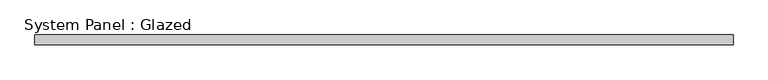
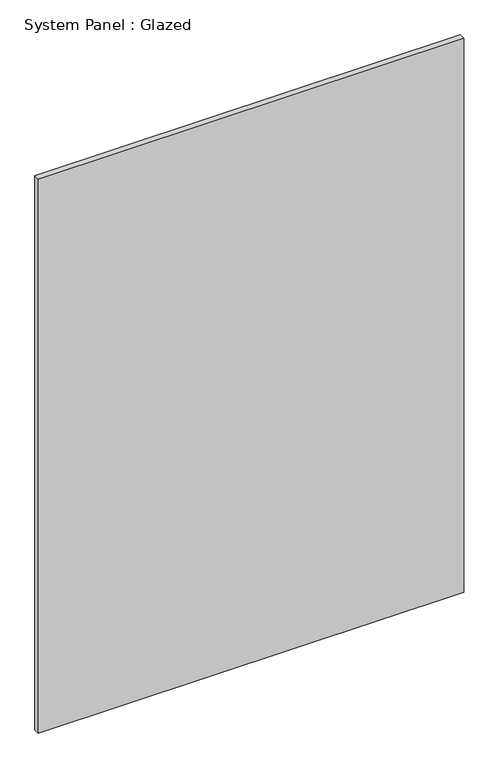
"""IFC4 building model written with IfcOpenShell, lengths in millimetres: plate geometry, System Panel : Glazed."""

import ifcopenshell
import ifcopenshell.guid

model = None  # the IFC model being written
_history = None  # IfcOwnerHistory: only IFC2X3 demands one
_inside = {}  # id of a spatial element -> (the spatial element, [elements in it])
_under = {}  # id of a project, library or spatial element -> (it, [spatial elements below it])
_declared = {}  # id of a project -> (the project, [libraries it declares])
_typed = {}  # id of a type object -> (the type object, [elements of that type])
_made_of = {}  # id of a material, layer set ... -> (it, [elements and type objects made of it])


def new_model(schema):
    """Start an empty IFC model of exactly this schema.

    Asked for "IFC4X3", IfcOpenShell would pick the latest addendum, in which some entities
    have other attributes; the version numbers below select the first issue.
    IFC2X3 requires an IfcOwnerHistory on every rooted entity: one is made here for all.
    """
    global model, _history
    if schema == "IFC4X3":
        model = ifcopenshell.file(schema_version=(4, 3, 0, 0))
    else:
        model = ifcopenshell.file(schema=schema)
    _inside.clear()
    _under.clear()
    _declared.clear()
    _typed.clear()
    _made_of.clear()
    _history = None
    if model.schema == "IFC2X3":
        org = make("IfcOrganization", Name="unknown")
        user = make(
            "IfcPersonAndOrganization",
            ThePerson=make("IfcPerson", FamilyName="unknown"),
            TheOrganization=org,
        )
        app = make(
            "IfcApplication",
            ApplicationDeveloper=org,
            Version="unknown",
            ApplicationFullName="unknown",
            ApplicationIdentifier="unknown",
        )
        _history = make(
            "IfcOwnerHistory",
            OwningUser=user,
            OwningApplication=app,
            ChangeAction="ADDED",
            CreationDate=0,
        )
    return model


def make(cls, **values):
    """One entity of the class cls with the attributes given. An attribute that is None is left unset."""
    return model.create_entity(
        cls, **{name: value for name, value in values.items() if value is not None}
    )


def rooted(cls, **values):
    """An entity with a GlobalId (a new one), such as an element, a storey or a relation."""
    return make(cls, GlobalId=ifcopenshell.guid.new(), OwnerHistory=_history, **values)


def si_unit(unit_type, name, prefix=None):
    """IfcSIUnit, for example si_unit("LENGTHUNIT", "METRE", prefix="MILLI")."""
    return make("IfcSIUnit", UnitType=unit_type, Prefix=prefix, Name=name)


def assignment(units):
    """IfcUnitAssignment: the units of a project."""
    return None if units is None else make("IfcUnitAssignment", Units=units)


def point(xyz):
    """IfcCartesianPoint."""
    return None if xyz is None else make("IfcCartesianPoint", Coordinates=xyz)


def direction(xyz):
    """IfcDirection."""
    return None if xyz is None else make("IfcDirection", DirectionRatios=xyz)


def frame(location, z_axis=None, x_axis=None):
    """IfcAxis2Placement3D, a coordinate frame: its origin and axes. An axis left out is left unset."""
    return make(
        "IfcAxis2Placement3D",
        Location=point(location),
        Axis=direction(z_axis),
        RefDirection=direction(x_axis),
    )


def origin():
    """The frame at (0, 0, 0) with its axes left unset."""
    return frame((0.0, 0.0, 0.0))


def origin_with_axes():
    """The frame at (0, 0, 0) with the z axis (0, 0, 1) and the x axis (1, 0, 0) written out."""
    return frame((0.0, 0.0, 0.0), z_axis=(0.0, 0.0, 1.0), x_axis=(1.0, 0.0, 0.0))


def place(relative_to, where):
    """IfcLocalPlacement: puts the frame where relative to a parent placement (None: the world)."""
    return make(
        "IfcLocalPlacement", PlacementRelTo=relative_to, RelativePlacement=where
    )


def context(
    kind, dimensions, precision=None, world=None, true_north=None, identifier=None
):
    """IfcGeometricRepresentationContext, for example the 3D "Model" context."""
    return make(
        "IfcGeometricRepresentationContext",
        ContextIdentifier=identifier,
        ContextType=kind,
        CoordinateSpaceDimension=dimensions,
        Precision=precision,
        WorldCoordinateSystem=world,
        TrueNorth=true_north,
    )


def project(units=None, contexts=None):
    """IfcProject with its units and contexts."""
    return rooted(
        "IfcProject",
        Name="project",
        RepresentationContexts=contexts,
        UnitsInContext=assignment(units),
    )


def spatial(cls, under=None, at=None, **own):
    """A site, building, storey or space (cls), placed at a placement, below another one or the project."""
    s = rooted(cls, ObjectPlacement=at, **own)
    if under is not None:
        _under.setdefault(under.id(), (under, []))[1].append(s)
    return s


def polyline(points):
    """IfcPolyline through the points."""
    return make("IfcPolyline", Points=[point(p) for p in points])


def outline(outer, holes=None, kind="AREA"):
    """IfcArbitraryClosedProfileDef: a profile drawn as a closed curve; with holes, ...WithVoids."""
    if holes is None:
        return make("IfcArbitraryClosedProfileDef", ProfileType=kind, OuterCurve=outer)
    return make(
        "IfcArbitraryProfileDefWithVoids",
        ProfileType=kind,
        OuterCurve=outer,
        InnerCurves=holes,
    )


def extrude(swept, where, along, depth):
    """IfcExtrudedAreaSolid: the profile swept, set in the frame where, extruded along a direction by depth."""
    return make(
        "IfcExtrudedAreaSolid",
        SweptArea=swept,
        Position=where,
        ExtrudedDirection=direction(along),
        Depth=depth,
    )


def shape(context_of_items, identifier, shape_type, items):
    """IfcShapeRepresentation: the items that make up one representation, for example the "Body"."""
    return make(
        "IfcShapeRepresentation",
        ContextOfItems=context_of_items,
        RepresentationIdentifier=identifier,
        RepresentationType=shape_type,
        Items=items,
    )


def source(mapping_origin, context_of_items, identifier, shape_type, items):
    """IfcRepresentationMap: a shape defined once, which mapped items show again and again."""
    return make(
        "IfcRepresentationMap",
        MappingOrigin=mapping_origin,
        MappedRepresentation=shape(context_of_items, identifier, shape_type, items),
    )


def transform(
    local_origin,
    x_axis=None,
    y_axis=None,
    z_axis=None,
    scale=None,
    scale2=None,
    scale3=None,
    uniform=True,
):
    """IfcCartesianTransformationOperator3D, or its non-uniform kind. x_axis, y_axis, z_axis: its Axis1, 2, 3."""
    if uniform:
        return make(
            "IfcCartesianTransformationOperator3D",
            Axis1=direction(x_axis),
            Axis2=direction(y_axis),
            LocalOrigin=point(local_origin),
            Scale=scale,
            Axis3=direction(z_axis),
        )
    return make(
        "IfcCartesianTransformationOperator3DnonUniform",
        Axis1=direction(x_axis),
        Axis2=direction(y_axis),
        LocalOrigin=point(local_origin),
        Scale=scale,
        Axis3=direction(z_axis),
        Scale2=scale2,
        Scale3=scale3,
    )


def mapped(mapping_source, mapping_target):
    """IfcMappedItem: shows the shape of a source again, moved by a transform."""
    return make(
        "IfcMappedItem", MappingSource=mapping_source, MappingTarget=mapping_target
    )


def made_of(thing, what):
    """Note that an element or type object is made of a material, layer set ...; save() writes the relation."""
    if what is not None:
        _made_of.setdefault(what.id(), (what, []))[1].append(thing)
    return thing


def element(
    cls,
    number,
    at=None,
    inside=None,
    cuts=None,
    type_object=None,
    material=None,
    context=None,
    identifier="Body",
    shape_type=None,
    held_by="IfcProductDefinitionShape",
    body=None,
    shapes=None,
    **own,
):
    """One element of the class cls, such as IfcWall. Its Tag is "e" and its number.

    at: its placement. inside: the storey or other place that contains it. cuts: it is an
    opening in that element (IfcRelVoidsElement). A single representation is given by context,
    identifier, shape_type and body (its items); several are given by shapes. held_by: the class
    of the entity that holds the representations. save() writes the other relations.
    """
    e = rooted(cls, Tag="e%d" % number, ObjectPlacement=at, **own)
    if body is not None:
        shapes = [shape(context, identifier, shape_type, body)]
    if shapes is not None:
        e.Representation = make(held_by, Representations=shapes)
    if inside is not None:
        _inside.setdefault(inside.id(), (inside, []))[1].append(e)
    if cuts is not None:
        rooted(
            "IfcRelVoidsElement", RelatingBuildingElement=cuts, RelatedOpeningElement=e
        )
    if type_object is not None:
        _typed.setdefault(type_object.id(), (type_object, []))[1].append(e)
    return made_of(e, material)


def aggregate(whole, parts):
    """IfcRelAggregates: a whole, such as a stair, and the parts it consists of."""
    return rooted("IfcRelAggregates", RelatingObject=whole, RelatedObjects=parts)


def save(model, path):
    """Write the relations noted so far, then the file.

    IfcRelAggregates (storeys below a building ...), IfcRelContainedInSpatialStructure (elements
    in a storey), IfcRelDefinesByType, IfcRelAssociatesMaterial and IfcRelDeclares: one each for
    every whole, place, type object, material and project.
    """
    for whole, parts in _under.values():
        aggregate(whole, parts)
    for where, things in _inside.values():
        rooted(
            "IfcRelContainedInSpatialStructure",
            RelatedElements=things,
            RelatingStructure=where,
        )
    for kind, things in _typed.values():
        rooted("IfcRelDefinesByType", RelatedObjects=things, RelatingType=kind)
    for what, things in _made_of.values():
        rooted("IfcRelAssociatesMaterial", RelatedObjects=things, RelatingMaterial=what)
    for by, libraries in _declared.values():
        rooted("IfcRelDeclares", RelatingContext=by, RelatedDefinitions=libraries)
    model.write(path)


def system_panel_glazed_3dade0f0(model_context):
    return source(origin(), model_context, "Body", "SweptSolid", [
        extrude(outline(polyline([(890.0, 24.5), (-890.0, 24.5), (-890.0, 49.5), (890.0, 49.5), (890.0, 24.5)])), origin_with_axes(), (0.0, 0.0, 1.0), 2450.0),
    ])


if __name__ == "__main__":
    model = new_model("IFC4")
    model_context = context("Model", 3, world=origin())
    ifc_project = project(units=[si_unit("LENGTHUNIT", "METRE", prefix="MILLI")], contexts=[model_context])
    site = spatial("IfcSite", under=ifc_project)
    building = spatial("IfcBuilding", under=site)
    placement = place(None, origin())
    system_panel_glazed_shape = system_panel_glazed_3dade0f0(model_context)
    element("IfcPlate", 1, ObjectType="System Panel : Glazed", at=placement, inside=building, context=model_context, shape_type="MappedRepresentation", body=[
        mapped(system_panel_glazed_shape, transform((0.0, 0.0, 0.0), x_axis=(1.0, 0.0, 0.0), y_axis=(0.0, 1.0, 0.0), z_axis=(0.0, 0.0, 1.0))),
    ])
    save(model, "model.ifc")

# Revit data of these elements
# Project information
#   Project Issue Date = "Issue Date"
#   Project Status = "Project Status"
#   Project Address = "Enter address here"
#   Project Name = "MASS BUILDING"
#   Project Number = "Project Number"
# Type "System Panel : Glazed"
#   Keynote = "H11"
#   Construction Type Id = "GSP4R"
#   Analytic Construction = "1/8 in Pilkington single glazing"
#   Visual Light Transmittance = 0.9
#   Solar Heat Gain Coefficient = 0.86
#   Heat Transfer Coefficient (U) = 6.7069 W/(m²·K)
# Element 1 (IfcPlate, "System Panel : Glazed")
#   Materials on its faces: "Glass"
# Materials
#   "Glass": class "Glass", colour RGB 0 128 192, transparency 0.9, Description = "Soda Lime Glass", Cost = 0
